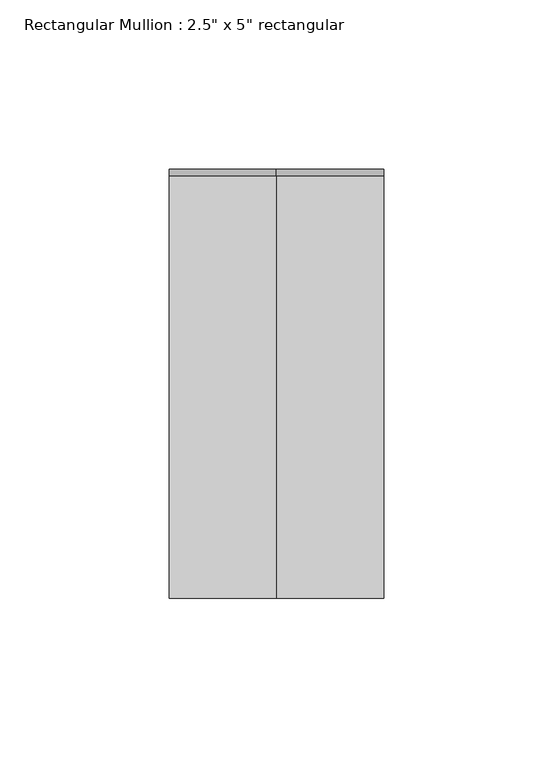
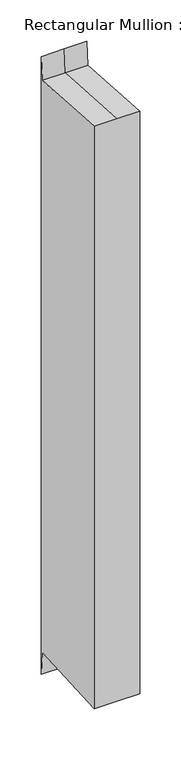
"""IFC4 building model written with IfcOpenShell, lengths in millimetres: member geometry."""

from ifc_helpers import new_model, si_unit, origin, place, context, project, spatial, faceted_brep, source, transform, mapped, element, save


def member_d702d02f(model_context):
    return source(origin(), model_context, "Body", "Brep", [
        faceted_brep([(-31.75, 63.5, 29.7846233), (0.0, 63.5, 29.7846233), (31.75, 63.5, 29.7846233), (31.75, 63.5, -880.6846233), (0.0, 63.5, -880.6846233), (-31.75, 63.5, -880.6846233), (-31.75, -63.5, 3.8736342), (-31.75, 61.4149606, -3.8662198), (-31.75, 61.4149606, -847.0337802), (-31.75, -63.5, -854.7736342), (31.75, -63.5, 3.8736342), (0.0, -63.5, 3.8736342), (0.0, -63.5, -854.7736342), (31.75, -63.5, -854.7736342), (31.75, 61.4149606, -3.8662198), (31.75, 61.4149606, -847.0337802), (0.0, 61.4149606, -3.8662198), (0.0, 61.4149606, -847.0337802)], [[[0, 1, 2, 3, 4, 5]], [[6, 7, 0, 5, 8, 9]], [[10, 11, 6, 9, 12, 13]], [[2, 14, 10, 13, 15, 3]], [[2, 1, 16, 14]], [[1, 0, 7, 16]], [[7, 6, 11, 16]], [[11, 10, 14, 16]], [[3, 15, 17, 4]], [[15, 13, 12, 17]], [[12, 9, 8, 17]], [[8, 5, 4, 17]]]),
    ])


if __name__ == "__main__":
    model = new_model("IFC4")
    model_context = context("Model", 3, world=origin())
    ifc_project = project(units=[si_unit("LENGTHUNIT", "METRE", prefix="MILLI")], contexts=[model_context])
    site = spatial("IfcSite", under=ifc_project)
    building = spatial("IfcBuilding", under=site)
    placement = place(None, origin())
    member_shape = member_d702d02f(model_context)
    element("IfcMember", 1, ObjectType="Rectangular Mullion : 2.5\" x 5\" rectangular", at=placement, inside=building, context=model_context, shape_type="MappedRepresentation", body=[
        mapped(member_shape, transform((0.0, 0.0, 0.0), x_axis=(1.0, 0.0, 0.0), y_axis=(0.0, 1.0, 0.0), z_axis=(0.0, 0.0, 1.0))),
    ])
    save(model, "model.ifc")

# Revit data of these elements
# Type "Rectangular Mullion : 2.5\" x 5\" rectangular"
#   built-in parameter 1007304 = 0.416667 (stored number, unit not read)
#   built-in parameter 1007301 = 0.104167 (stored number, unit not read)
#   built-in parameter 1007300 = 0.104167 (stored number, unit not read)
# Element 1 (IfcMember, "Rectangular Mullion : 2.5\" x 5\" rectangular")
#   Materials on its faces: "Metal - Aluminum"
# Materials
#   "Metal - Aluminum": class "Metal", colour RGB 247 247 247, transparency 0, Cost = 0
